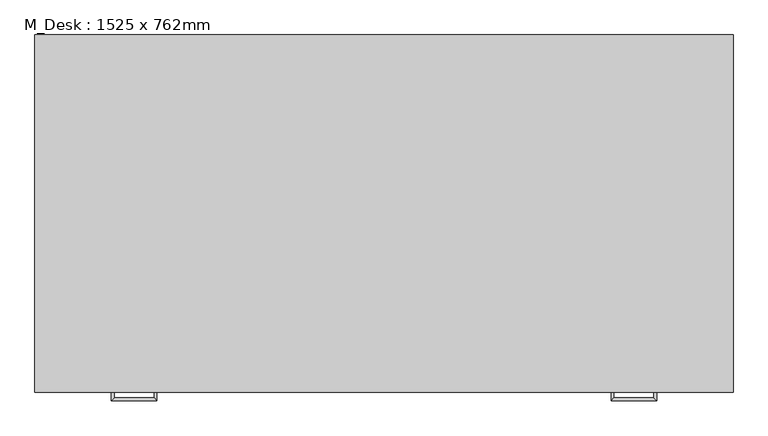
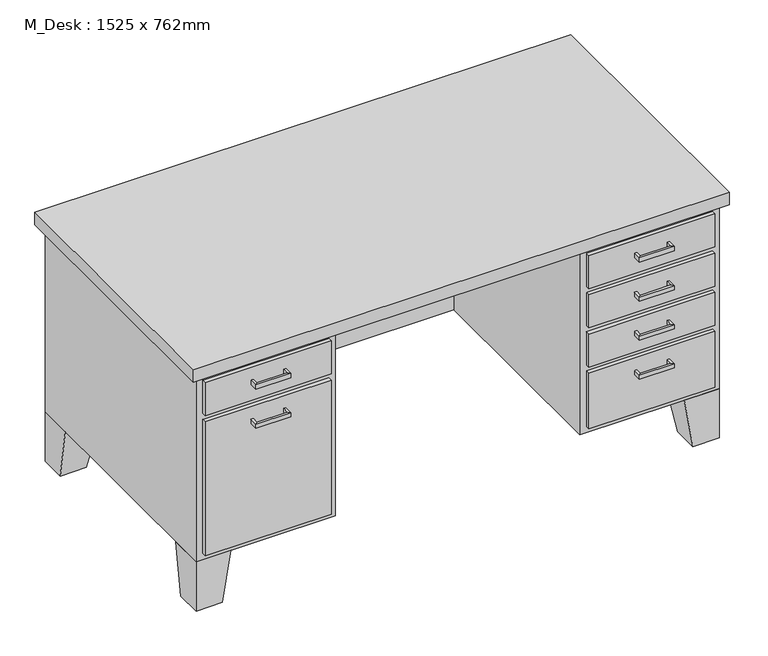
"""IFC4 building model written with IfcOpenShell, lengths in millimetres: furniture geometry, M_Desk : 1525 x 762mm."""

from ifc_helpers import new_model, si_unit, frame, origin, place, context, project, spatial, polyline, outline, extrude, faceted_brep, source, transform, mapped, element, save


def m_desk_1525_x_762mm_34485ced(model_context):
    return source(origin(), model_context, "Body", "SolidModel", [
        extrude(outline(polyline([(1118.1, 0.0), (1118.1, 635.0), (405.9, 635.0), (405.9, 0.0), (-0.5, 0.0), (-0.5, 762.0), (1524.5, 762.0), (1524.5, 0.0), (1118.1, 0.0)])), frame((0.0, 0.0, 152.0), z_axis=(0.0, 0.0, 1.0), x_axis=(1.0, 0.0, 0.0)), (0.0, 0.0, 1.0), 571.9),
        extrude(outline(polyline([(-19.55, -19.05), (-19.55, 781.05), (1543.55, 781.05), (1543.55, -19.05), (-19.55, -19.05)])), frame((0.0, 0.0, 723.9), z_axis=(0.0, 0.0, 1.0), x_axis=(1.0, 0.0, 0.0)), (0.0, 0.0, 1.0), 38.1),
        faceted_brep([(1422.9, 0.0, 152.0), (1524.5, 0.0, 152.0), (1524.5, 101.6, 152.0), (1422.9, 101.6, 152.0), (1448.3, 0.0, 0.0), (1448.3, 76.2, 0.0), (1524.5, 76.2, 0.0), (1524.5, 0.0, 0.0)], [[[0, 1, 2, 3]], [[4, 5, 6, 7]], [[4, 7, 1, 0]], [[7, 6, 2, 1]], [[6, 5, 3, 2]], [[5, 4, 0, 3]]]),
        faceted_brep([(1422.9, 762.0, 152.0), (1422.9, 660.4, 152.0), (1524.5, 660.4, 152.0), (1524.5, 762.0, 152.0), (1448.3, 762.0, 0.0), (1524.5, 762.0, 0.0), (1524.5, 685.8, 0.0), (1448.3, 685.8, 0.0)], [[[0, 1, 2, 3]], [[4, 5, 6, 7]], [[4, 7, 1, 0]], [[7, 6, 2, 1]], [[6, 5, 3, 2]], [[5, 4, 0, 3]]]),
        faceted_brep([(101.1, 762.0, 152.0), (-0.5, 762.0, 152.0), (-0.5, 660.4, 152.0), (101.1, 660.4, 152.0), (75.7, 762.0, 0.0), (75.7, 685.8, 0.0), (-0.5, 685.8, 0.0), (-0.5, 762.0, 0.0)], [[[0, 1, 2, 3]], [[4, 5, 6, 7]], [[4, 7, 1, 0]], [[7, 6, 2, 1]], [[6, 5, 3, 2]], [[5, 4, 0, 3]]]),
        faceted_brep([(101.1, 0.0, 152.0), (101.1, 101.6, 152.0), (-0.5, 101.6, 152.0), (-0.5, 0.0, 152.0), (75.7, 0.0, 0.0), (-0.5, 0.0, 0.0), (-0.5, 76.2, 0.0), (75.7, 76.2, 0.0)], [[[0, 1, 2, 3]], [[4, 5, 6, 7]], [[4, 7, 1, 0]], [[7, 6, 2, 1]], [[6, 5, 3, 2]], [[5, 4, 0, 3]]]),
        extrude(outline(polyline([(1137.15, 0.0), (1505.45, 0.0), (1505.45, -12.7), (1137.15, -12.7), (1137.15, 0.0)])), frame((0.0, 0.0, 602.85), z_axis=(0.0, 0.0, 1.0), x_axis=(1.0, 0.0, 0.0)), (0.0, 0.0, 1.0), 102.0),
        extrude(outline(polyline([(1137.15, 0.0), (1505.45, 0.0), (1505.45, -12.7), (1137.15, -12.7), (1137.15, 0.0)])), frame((0.0, 0.0, 171.05), z_axis=(0.0, 0.0, 1.0), x_axis=(1.0, 0.0, 0.0)), (0.0, 0.0, 1.0), 171.45),
        extrude(outline(polyline([(1137.15, 0.0), (1505.45, 0.0), (1505.45, -12.7), (1137.15, -12.7), (1137.15, 0.0)])), frame((0.0, 0.0, 482.2), z_axis=(0.0, 0.0, 1.0), x_axis=(1.0, 0.0, 0.0)), (0.0, 0.0, 1.0), 101.6),
        extrude(outline(polyline([(1137.15, 0.0), (1505.45, 0.0), (1505.45, -12.7), (1137.15, -12.7), (1137.15, 0.0)])), frame((0.0, 0.0, 361.55), z_axis=(0.0, 0.0, 1.0), x_axis=(1.0, 0.0, 0.0)), (0.0, 0.0, 1.0), 101.6),
        extrude(outline(polyline([(18.55, 0.0), (386.85, 0.0), (386.85, -12.7), (18.55, -12.7), (18.55, 0.0)])), frame((0.0, 0.0, 603.25), z_axis=(0.0, 0.0, 1.0), x_axis=(1.0, 0.0, 0.0)), (0.0, 0.0, 1.0), 101.6),
        extrude(outline(polyline([(18.55, 0.0), (386.85, 0.0), (386.85, -12.7), (18.55, -12.7), (18.55, 0.0)])), frame((0.0, 0.0, 171.05), z_axis=(0.0, 0.0, 1.0), x_axis=(1.0, 0.0, 0.0)), (0.0, 0.0, 1.0), 413.15),
        faceted_brep([(1365.75, -12.7, 304.8), (1372.1, -12.7, 304.8), (1372.1, -12.7, 292.1), (1365.75, -12.7, 292.1), (1365.75, -31.75, 304.8), (1372.1, -38.1, 304.8), (1372.1, -38.1, 292.1), (1365.75, -31.75, 292.1), (1276.85, -31.75, 304.8), (1270.5, -38.1, 304.8), (1270.5, -38.1, 292.1), (1276.85, -31.75, 292.1), (1276.85, -12.7, 304.8), (1276.85, -12.7, 292.1), (1270.5, -12.7, 292.1), (1270.5, -12.7, 304.8)], [[[0, 1, 2, 3]], [[1, 0, 4, 5]], [[2, 1, 5, 6]], [[3, 2, 6, 7]], [[0, 3, 7, 4]], [[5, 4, 8, 9]], [[6, 5, 9, 10]], [[7, 6, 10, 11]], [[4, 7, 11, 8]], [[12, 13, 14, 15]], [[9, 8, 12, 15]], [[10, 9, 15, 14]], [[11, 10, 14, 13]], [[8, 11, 13, 12]]]),
        faceted_brep([(1365.75, -12.7, 425.45), (1372.1, -12.7, 425.45), (1372.1, -12.7, 412.75), (1365.75, -12.7, 412.75), (1365.75, -31.75, 425.45), (1372.1, -38.1, 425.45), (1372.1, -38.1, 412.75), (1365.75, -31.75, 412.75), (1276.85, -31.75, 425.45), (1270.5, -38.1, 425.45), (1270.5, -38.1, 412.75), (1276.85, -31.75, 412.75), (1276.85, -12.7, 425.45), (1276.85, -12.7, 412.75), (1270.5, -12.7, 412.75), (1270.5, -12.7, 425.45)], [[[0, 1, 2, 3]], [[1, 0, 4, 5]], [[2, 1, 5, 6]], [[3, 2, 6, 7]], [[0, 3, 7, 4]], [[5, 4, 8, 9]], [[6, 5, 9, 10]], [[7, 6, 10, 11]], [[4, 7, 11, 8]], [[12, 13, 14, 15]], [[9, 8, 12, 15]], [[10, 9, 15, 14]], [[11, 10, 14, 13]], [[8, 11, 13, 12]]]),
        faceted_brep([(1365.75, -12.7, 546.1), (1372.1, -12.7, 546.1), (1372.1, -12.7, 533.4), (1365.75, -12.7, 533.4), (1365.75, -31.75, 546.1), (1372.1, -38.1, 546.1), (1372.1, -38.1, 533.4), (1365.75, -31.75, 533.4), (1276.85, -31.75, 546.1), (1270.5, -38.1, 546.1), (1270.5, -38.1, 533.4), (1276.85, -31.75, 533.4), (1276.85, -12.7, 546.1), (1276.85, -12.7, 533.4), (1270.5, -12.7, 533.4), (1270.5, -12.7, 546.1)], [[[0, 1, 2, 3]], [[1, 0, 4, 5]], [[2, 1, 5, 6]], [[3, 2, 6, 7]], [[0, 3, 7, 4]], [[5, 4, 8, 9]], [[6, 5, 9, 10]], [[7, 6, 10, 11]], [[4, 7, 11, 8]], [[12, 13, 14, 15]], [[9, 8, 12, 15]], [[10, 9, 15, 14]], [[11, 10, 14, 13]], [[8, 11, 13, 12]]]),
        faceted_brep([(1365.75, -12.7, 666.75), (1372.1, -12.7, 666.75), (1372.1, -12.7, 654.05), (1365.75, -12.7, 654.05), (1365.75, -31.75, 666.75), (1372.1, -38.1, 666.75), (1372.1, -38.1, 654.05), (1365.75, -31.75, 654.05), (1276.85, -31.75, 666.75), (1270.5, -38.1, 666.75), (1270.5, -38.1, 654.05), (1276.85, -31.75, 654.05), (1276.85, -12.7, 666.75), (1276.85, -12.7, 654.05), (1270.5, -12.7, 654.05), (1270.5, -12.7, 666.75)], [[[0, 1, 2, 3]], [[1, 0, 4, 5]], [[2, 1, 5, 6]], [[3, 2, 6, 7]], [[0, 3, 7, 4]], [[5, 4, 8, 9]], [[6, 5, 9, 10]], [[7, 6, 10, 11]], [[4, 7, 11, 8]], [[12, 13, 14, 15]], [[9, 8, 12, 15]], [[10, 9, 15, 14]], [[11, 10, 14, 13]], [[8, 11, 13, 12]]]),
        faceted_brep([(158.25, -12.7, 546.1), (158.25, -12.7, 533.4), (151.9, -12.7, 533.4), (151.9, -12.7, 546.1), (158.25, -31.75, 546.1), (158.25, -31.75, 533.4), (151.9, -38.1, 533.4), (151.9, -38.1, 546.1), (247.15, -31.75, 546.1), (247.15, -31.75, 533.4), (253.5, -38.1, 533.4), (253.5, -38.1, 546.1), (247.15, -12.7, 546.1), (253.5, -12.7, 546.1), (253.5, -12.7, 533.4), (247.15, -12.7, 533.4)], [[[0, 1, 2, 3]], [[1, 0, 4, 5]], [[2, 1, 5, 6]], [[3, 2, 6, 7]], [[0, 3, 7, 4]], [[5, 4, 8, 9]], [[6, 5, 9, 10]], [[7, 6, 10, 11]], [[4, 7, 11, 8]], [[12, 13, 14, 15]], [[9, 8, 12, 15]], [[10, 9, 15, 14]], [[11, 10, 14, 13]], [[8, 11, 13, 12]]]),
        faceted_brep([(158.25, -12.7, 666.75), (158.25, -12.7, 654.05), (151.9, -12.7, 654.05), (151.9, -12.7, 666.75), (158.25, -31.75, 666.75), (158.25, -31.75, 654.05), (151.9, -38.1, 654.05), (151.9, -38.1, 666.75), (247.15, -31.75, 666.75), (247.15, -31.75, 654.05), (253.5, -38.1, 654.05), (253.5, -38.1, 666.75), (247.15, -12.7, 666.75), (253.5, -12.7, 666.75), (253.5, -12.7, 654.05), (247.15, -12.7, 654.05)], [[[0, 1, 2, 3]], [[1, 0, 4, 5]], [[2, 1, 5, 6]], [[3, 2, 6, 7]], [[0, 3, 7, 4]], [[5, 4, 8, 9]], [[6, 5, 9, 10]], [[7, 6, 10, 11]], [[4, 7, 11, 8]], [[12, 13, 14, 15]], [[9, 8, 12, 15]], [[10, 9, 15, 14]], [[11, 10, 14, 13]], [[8, 11, 13, 12]]]),
    ])


if __name__ == "__main__":
    model = new_model("IFC4")
    model_context = context("Model", 3, world=origin())
    ifc_project = project(units=[si_unit("LENGTHUNIT", "METRE", prefix="MILLI")], contexts=[model_context])
    site = spatial("IfcSite", under=ifc_project)
    building = spatial("IfcBuilding", under=site)
    placement = place(None, origin())
    m_desk_1525_x_762mm_shape = m_desk_1525_x_762mm_34485ced(model_context)
    element("IfcFurniture", 1, ObjectType="M_Desk : 1525 x 762mm", at=placement, inside=building, context=model_context, shape_type="MappedRepresentation", body=[
        mapped(m_desk_1525_x_762mm_shape, transform((0.0, 0.0, 0.0), x_axis=(1.0, 0.0, 0.0), y_axis=(0.0, 1.0, 0.0), z_axis=(0.0, 0.0, 1.0))),
    ])
    save(model, "model.ifc")

# Revit data of these elements
# Type "M_Desk : 1525 x 762mm"
#   Depth = 762 mm
#   Height = 762 mm
#   Leg Height = 152 mm
#   Width = 1525 mm
#   Body Material = Laminate, Ivory, Matte
#   Handle/Leg Material = Steel, Chrome Plated
#   Top Material = Cherry
#   Default Elevation = 0
#   Assembly Code = ""
# Element 1 (IfcFurniture, "M_Desk : 1525 x 762mm")
#   Materials on its faces: "Steel, Chrome Plated", "Laminate, Ivory, Matte", "Cherry"
# Materials
#   "Laminate, Ivory, Matte": class "Plastic", colour RGB 244 244 244, transparency 0, Description = "Plastic Laminate - Ivory, Matte", Cost = 0
#   "Steel, Chrome Plated": class "Metal", colour RGB 17 17 17, transparency 0, Description = "Chromiuim plated steel", Cost = 0
#   "Cherry": class "Wood", colour RGB 158 77 40, transparency 0, Description = "Prunus Serotina", Cost = 0
